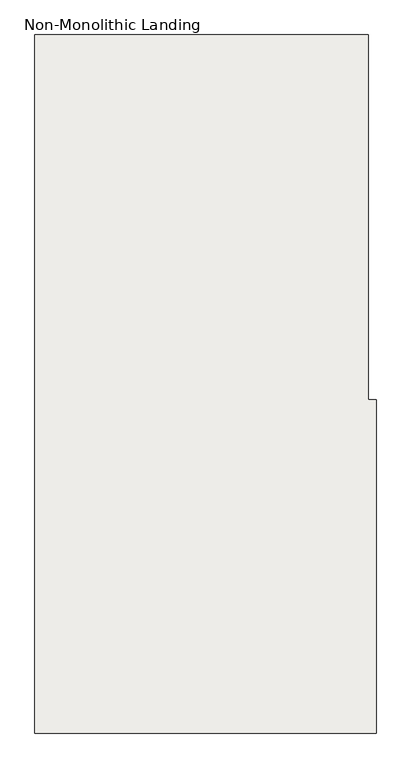
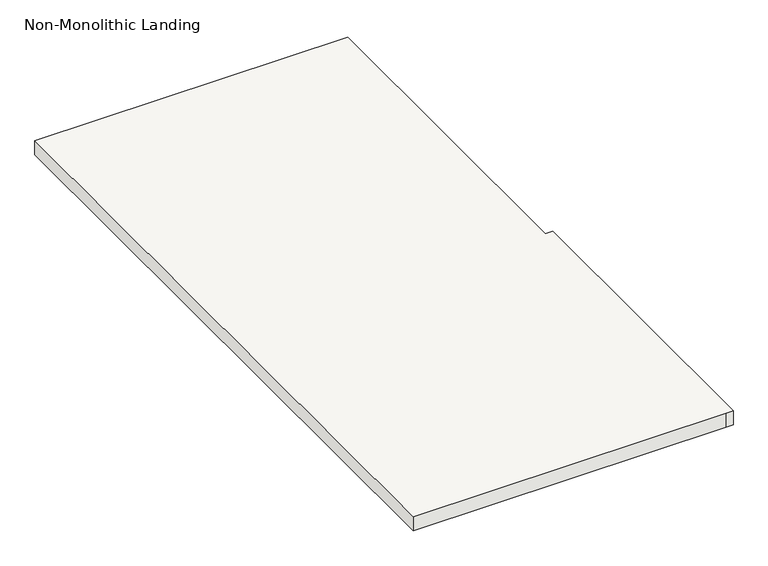
"""IFC4 building model written with IfcOpenShell, lengths in millimetres: slab geometry, Non-Monolithic Landing."""

from ifc_helpers import new_model, si_unit, origin, place, context, project, spatial, faceted_brep, source, transform, mapped, element, save


def non_monolithic_landing_082eb450(model_context):
    return source(origin(), model_context, "Body", "Brep", [
        faceted_brep([(663695.788677, -549416.0413841, 3143.5932432), (663721.188677, -549416.0413841, 3168.9932432), (663721.188677, -550482.8413841, 3168.9932432), (663695.788677, -550482.8413841, 3143.5932432), (662654.388677, -549416.0413841, 3188.0432432), (662654.388677, -551651.2413841, 3188.0432432), (663721.188677, -551651.2413841, 3188.0432432), (663746.588677, -551651.2413841, 3188.0432432), (663746.588677, -550584.4413841, 3188.0432432), (663721.188677, -550584.4413841, 3188.0432432), (663721.188677, -549416.0413841, 3188.0432432), (663695.788677, -550482.8413841, 3137.2432432), (663721.188677, -550482.8413841, 3137.2432432), (663721.188677, -550584.4413841, 3137.2432432), (663746.588677, -550584.4413841, 3137.2432432), (663746.588677, -551651.2413841, 3137.2432432), (663721.188677, -551651.2413841, 3137.2432432), (662654.388677, -551651.2413841, 3137.2432432), (662654.388677, -549416.0413841, 3137.2432432), (663695.788677, -549416.0413841, 3137.2432432)], [[[0, 1, 2, 3]], [[4, 5, 6, 7, 8, 9, 10]], [[11, 12, 13, 14, 15, 16, 17, 18, 19]], [[12, 11, 3, 2]], [[11, 19, 0, 3]], [[4, 10, 1, 0, 19, 18]], [[5, 4, 18, 17]], [[6, 5, 17, 16]], [[7, 6, 16, 15]], [[8, 7, 15, 14]], [[9, 8, 14, 13]], [[10, 9, 13, 12, 2, 1]]]),
    ])


if __name__ == "__main__":
    model = new_model("IFC4")
    model_context = context("Model", 3, world=origin())
    ifc_project = project(units=[si_unit("LENGTHUNIT", "METRE", prefix="MILLI")], contexts=[model_context])
    site = spatial("IfcSite", under=ifc_project)
    building = spatial("IfcBuilding", under=site)
    placement = place(None, origin())
    non_monolithic_landing_shape = non_monolithic_landing_082eb450(model_context)
    element("IfcSlab", 1, ObjectType="Non-Monolithic Landing", at=placement, inside=building, context=model_context, shape_type="MappedRepresentation", body=[
        mapped(non_monolithic_landing_shape, transform((0.0, 0.0, 0.0), x_axis=(1.0, 0.0, 0.0), y_axis=(0.0, 1.0, 0.0), z_axis=(0.0, 0.0, 1.0))),
    ])
    save(model, "model.ifc")
